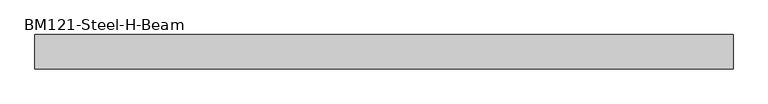
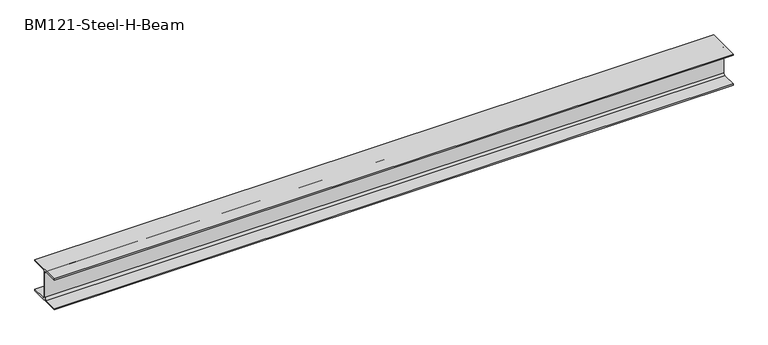
"""IFC4 building model written with IfcOpenShell, lengths in millimetres: beam geometry, BM121-Steel-H-Beam : BM121_H-294×302x12x12."""

from ifc_helpers import new_model, si_unit, point, frame, frame_2d, origin, place, context, project, spatial, polyline, circle_curve, trimmed, segment, composite_curve, outline, extrude, source, transform, mapped, element, save


def bm121_steel_h_beam_5f4759b5(model_context):
    return source(origin(), model_context, "Body", "SweptSolid", [
        extrude(outline(composite_curve([segment(polyline([(151.0, 147.0), (151.0, 135.0), (24.0, 135.0)]), True, "CONTINUOUS"), segment(trimmed(circle_curve(frame_2d((24.0, 117.0)), 18.0), [point((24.0, 135.0))], [point((6.0, 117.0))], True, "CARTESIAN"), True, "CONTINUOUS"), segment(polyline([(6.0, 117.0), (6.0, -117.0)]), True, "CONTINUOUS"), segment(trimmed(circle_curve(frame_2d((24.0, -117.0)), 18.0), [point((6.0, -117.0))], [point((24.0, -135.0))], True, "CARTESIAN"), True, "CONTINUOUS"), segment(polyline([(24.0, -135.0), (151.0, -135.0), (151.0, -147.0), (-151.0, -147.0), (-151.0, -135.0), (-24.0, -135.0)]), True, "CONTINUOUS"), segment(trimmed(circle_curve(frame_2d((-24.0, -117.0)), 18.0), [point((-24.0, -135.0))], [point((-6.0, -117.0))], True, "CARTESIAN"), True, "CONTINUOUS"), segment(polyline([(-6.0, -117.0), (-6.0, 117.0)]), True, "CONTINUOUS"), segment(trimmed(circle_curve(frame_2d((-24.0, 117.0)), 18.0), [point((-6.0, 117.0))], [point((-24.0, 135.0))], True, "CARTESIAN"), True, "CONTINUOUS"), segment(polyline([(-24.0, 135.0), (-151.0, 135.0), (-151.0, 147.0), (151.0, 147.0)]), True, "CONTINUOUS")], self_intersect=False)), frame((-3130.5756627, 0.0, 0.0), z_axis=(1.0, 0.0, 0.0), x_axis=(0.0, 1.0, 0.0)), (0.0, 0.0, 1.0), 6100.2),
    ])


if __name__ == "__main__":
    model = new_model("IFC4")
    model_context = context("Model", 3, world=origin())
    ifc_project = project(units=[si_unit("LENGTHUNIT", "METRE", prefix="MILLI")], contexts=[model_context])
    site = spatial("IfcSite", under=ifc_project)
    building = spatial("IfcBuilding", under=site)
    placement = place(None, origin())
    bm121_steel_h_beam_shape = bm121_steel_h_beam_5f4759b5(model_context)
    element("IfcBeam", 1, ObjectType="BM121-Steel-H-Beam : BM121_H-294×302x12x12", at=placement, inside=building, context=model_context, shape_type="MappedRepresentation", body=[
        mapped(bm121_steel_h_beam_shape, transform((0.0, 0.0, 0.0), x_axis=(1.0, 0.0, 0.0), y_axis=(0.0, 1.0, 0.0), z_axis=(0.0, 0.0, 1.0))),
    ])
    save(model, "model.ifc")

# Revit data of these elements
# Type "BM121-Steel-H-Beam : BM121_H-294×302x12x12"
#   tw = 12 mm
#   tf = 12 mm
#   r = 18 mm
#   bf = 302 mm
#   Unit Weight = 84.50 kg/m
#   Surface Area = 1.7411 m²/m
#   Length [instance default] = 3000 mm
#   H = 294 mm
#   Sectional Area = 10770.0 cm²
